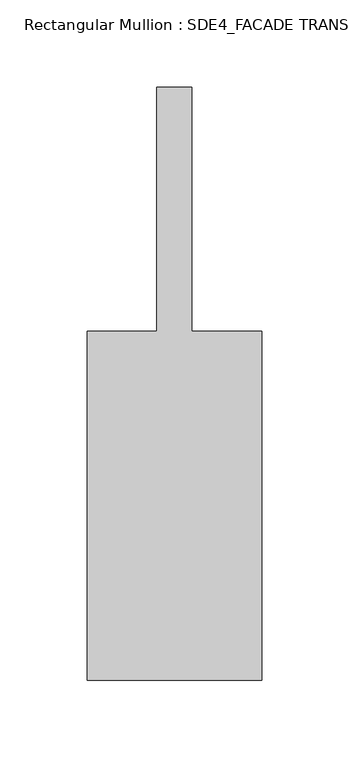
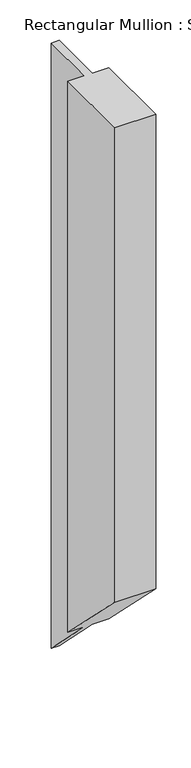
"""IFC4 building model written with IfcOpenShell, lengths in millimetres: member geometry, Rectangular Mullion : SDE4_FACADE TRANSOM TYPE 1."""

from ifc_helpers import new_model, si_unit, origin, place, context, project, spatial, faceted_brep, source, transform, mapped, element, save


def rectangular_mullion_sde4_facade_transom_type_1_01765e42(model_context):
    return source(origin(), model_context, "Body", "Brep", [
        faceted_brep([(50.0, -132.5, 0.0), (50.0, 67.5, 0.0), (10.0, 67.5, 0.0), (10.0, 207.5, 0.0), (-10.0, 207.5, 0.0), (-10.0, 67.5, 0.0), (-50.0, 67.5, 0.0), (-50.0, -132.5, 0.0), (50.0, -132.5, -1230.3200128), (50.0, 67.5, -1430.3200128), (10.0, 67.5, -1430.3200128), (10.0, 207.5, -1570.3200128), (-10.0, 207.5, -1570.3200128), (-10.0, 67.5, -1430.3200128), (-50.0, 67.5, -1430.3200128), (-50.0, -132.5, -1230.3200128)], [[[0, 1, 2, 3, 4, 5, 6, 7]], [[1, 0, 8, 9]], [[2, 1, 9, 10]], [[3, 2, 10, 11]], [[4, 3, 11, 12]], [[5, 4, 12, 13]], [[6, 5, 13, 14]], [[7, 6, 14, 15]], [[0, 7, 15, 8]], [[8, 15, 14, 13, 12, 11, 10, 9]]]),
    ])


if __name__ == "__main__":
    model = new_model("IFC4")
    model_context = context("Model", 3, world=origin())
    ifc_project = project(units=[si_unit("LENGTHUNIT", "METRE", prefix="MILLI")], contexts=[model_context])
    site = spatial("IfcSite", under=ifc_project)
    building = spatial("IfcBuilding", under=site)
    placement = place(None, origin())
    rectangular_mullion_sde4_facade_transom_type_1_shape = rectangular_mullion_sde4_facade_transom_type_1_01765e42(model_context)
    element("IfcMember", 1, ObjectType="Rectangular Mullion : SDE4_FACADE TRANSOM TYPE 1", at=placement, inside=building, context=model_context, shape_type="MappedRepresentation", body=[
        mapped(rectangular_mullion_sde4_facade_transom_type_1_shape, transform((0.0, 0.0, 0.0), x_axis=(1.0, 0.0, 0.0), y_axis=(0.0, 1.0, 0.0), z_axis=(0.0, 0.0, 1.0))),
    ])
    save(model, "model.ifc")

# Revit data of these elements
# Project information
#   BLK No = "adqaa"
#   Project Name 2 = "SK N4C20"
#   Author = "XXX"
#   Job Title = "SENGKANG NEIGHBOURHOOD 4 CONTRACT 20"
#   Lot No = "XXX"
#   Mukim No = "XXX"
#   DSG 1 = "XXX"
#   DSG 2 = "XXX"
#   HDB Drawing No = "HB-D000-AR-"
#   Drawing No = "SB-DP-XXXX-D000-AR-"
#   Designation = "XXX"
#   Design Option = "Main Model"
#   Precinct Name = "XXXX"
#   Project Issue Date = "AUG 2016"
#   Project Status = "Project Status"
#   Client Name = "Owner"
#   Project Address = "Enter address here"
#   Project Name = "SENGKANG NEIGHBOURHOOD 4 CONTRACT 20"
#   Project Number = "A1952-00002-2014 BP01"
# Type "Rectangular Mullion : SDE4_FACADE TRANSOM TYPE 1"
#   built-in parameter 1007322 = 1.11549 (stored number, unit not read)
#   built-in parameter 1007321 = 0.164042 (stored number, unit not read)
#   built-in parameter 1007320 = 0.164042 (stored number, unit not read)
